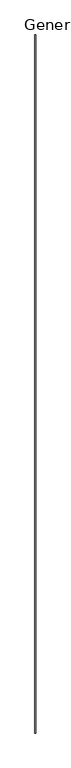
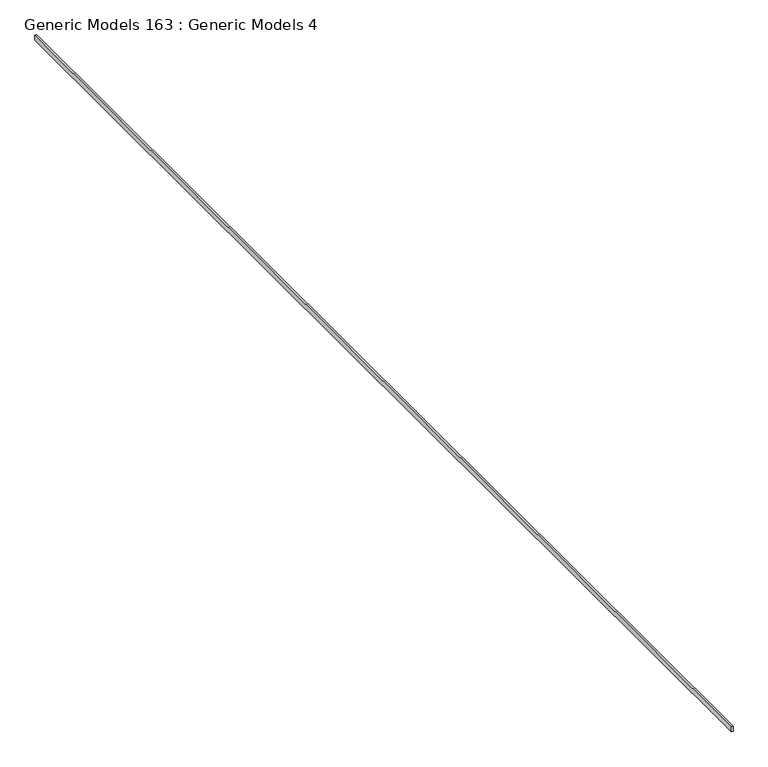
"""IFC4 building model written with IfcOpenShell, lengths in millimetres: proxy geometry, Generic Models 163 : Generic Models 4."""

from ifc_helpers import new_model, si_unit, frame, origin, place, context, project, spatial, polyline, outline, extrude, source, transform, mapped, element, save


def generic_models_163_generic_models_4_c4fb09a0(model_context):
    return source(origin(), model_context, "Body", "SweptSolid", [
        extrude(outline(polyline([(-10236.1097239, -5493.3230338), (-10252.9339552, -5493.3230338), (-10252.9339552, 7054.2769662), (-10236.1097239, 7054.2769662), (-10236.1097239, -5493.3230338)])), frame((0.0, 0.0, 122784.1984874), z_axis=(0.0, 0.0, 1.0), x_axis=(1.0, 0.0, 0.0)), (0.0, 0.0, 1.0), 54.2029547),
    ])


if __name__ == "__main__":
    model = new_model("IFC4")
    model_context = context("Model", 3, world=origin())
    ifc_project = project(units=[si_unit("LENGTHUNIT", "METRE", prefix="MILLI")], contexts=[model_context])
    site = spatial("IfcSite", under=ifc_project)
    building = spatial("IfcBuilding", under=site)
    placement = place(None, origin())
    generic_models_163_generic_models_4_shape = generic_models_163_generic_models_4_c4fb09a0(model_context)
    element("IfcBuildingElementProxy", 1, Name="Generic Models 163 : Generic Models 4", ObjectType="Generic Models 163 : Generic Models 4", at=placement, inside=building, context=model_context, shape_type="MappedRepresentation", body=[
        mapped(generic_models_163_generic_models_4_shape, transform((0.0, 0.0, 0.0), x_axis=(1.0, 0.0, 0.0), y_axis=(0.0, 1.0, 0.0), z_axis=(0.0, 0.0, 1.0))),
    ])
    save(model, "model.ifc")

# Revit data of these elements
# Element 1 (IfcBuildingElementProxy, "Generic Models 163 : Generic Models 4")
#   Materials on its faces: "_MORTAR SETTING BED"
# Materials
#   "_MORTAR SETTING BED": class "Generic", colour RGB 191 191 191, transparency 0, Cost = 0
